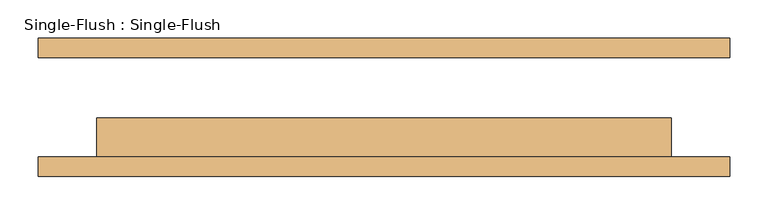
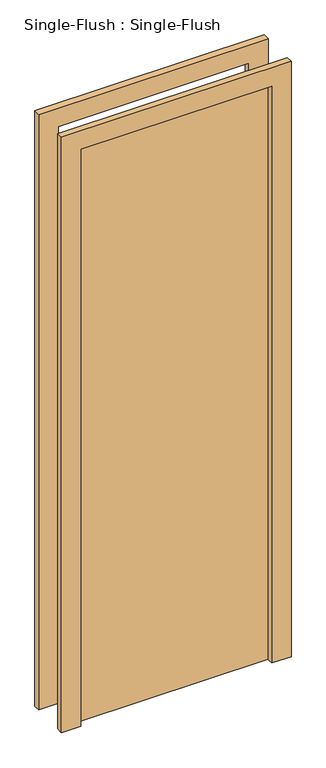
"""IFC4 building model written with IfcOpenShell, lengths in millimetres: door geometry, Single-Flush : Single-Flush."""

from ifc_helpers import new_model, si_unit, frame, origin, origin_with_axes, place, context, project, spatial, polyline, outline, extrude, source, transform, mapped, element, save


def single_flush_single_flush_4ef540a7(model_context):
    return source(origin(), model_context, "Body", "SweptSolid", [
        extrude(outline(polyline([(375.0, -14.2), (375.0, -65.0), (-375.0, -65.0), (-375.0, -14.2), (375.0, -14.2)])), origin_with_axes(), (0.0, 0.0, 1.0), 2400.0),
        extrude(outline(polyline([(2476.2, 451.2), (2476.2, -451.2), (0.0, -451.2), (0.0, -375.0), (2400.0, -375.0), (2400.0, 375.0), (0.0, 375.0), (0.0, 451.2), (2476.2, 451.2)])), frame((0.0, 65.0, 0.0), z_axis=(0.0, 1.0, 0.0), x_axis=(0.0, 0.0, 1.0)), (0.0, 0.0, 1.0), 25.4),
        extrude(outline(polyline([(2476.2, -451.2), (0.0, -451.2), (0.0, -375.0), (2400.0, -375.0), (2400.0, 375.0), (0.0, 375.0), (0.0, 451.2), (2476.2, 451.2), (2476.2, -451.2)])), frame((0.0, -90.4, 0.0), z_axis=(0.0, 1.0, 0.0), x_axis=(0.0, 0.0, 1.0)), (0.0, 0.0, 1.0), 25.4),
    ])


if __name__ == "__main__":
    model = new_model("IFC4")
    model_context = context("Model", 3, world=origin())
    ifc_project = project(units=[si_unit("LENGTHUNIT", "METRE", prefix="MILLI")], contexts=[model_context])
    site = spatial("IfcSite", under=ifc_project)
    building = spatial("IfcBuilding", under=site)
    placement = place(None, origin())
    single_flush_single_flush_shape = single_flush_single_flush_4ef540a7(model_context)
    element("IfcDoor", 1, ObjectType="Single-Flush : Single-Flush", at=placement, inside=building, context=model_context, shape_type="MappedRepresentation", body=[
        mapped(single_flush_single_flush_shape, transform((0.0, 0.0, 0.0), x_axis=(1.0, 0.0, 0.0), y_axis=(0.0, 1.0, 0.0), z_axis=(0.0, 0.0, 1.0))),
    ])
    save(model, "model.ifc")

# Revit data of these elements
# Type "Single-Flush : Single-Flush"
#   Type Mark = "61"
#   Assembly Code = "C1020"
#   Analytic Construction = "<None>"
#   Thickness = 50.8 mm
#   Height = 2400 mm
#   Trim Projection Ext = 25.4 mm
#   Trim Projection Int = 25.4 mm
#   Trim Width = 76.2 mm
#   Width = 750 mm
#   Define Thermal Properties by = 1
#   Door Material = Door - Panel
#   Frame Material = Door - Frame
#   Function = (empty or 0)
#   Wall Closure = (empty or 0)
# Element 1 (IfcDoor, "Single-Flush : Single-Flush")
#   Materials on its faces: "Door - Frame", "Door - Panel"
# Materials
#   "Door - Panel": class "Wood", colour RGB 210 159 95, transparency 0, Cost = 0
#   "Door - Frame": class "Unassigned", colour RGB 118 70 51, transparency 0, Keynote = "L20"
